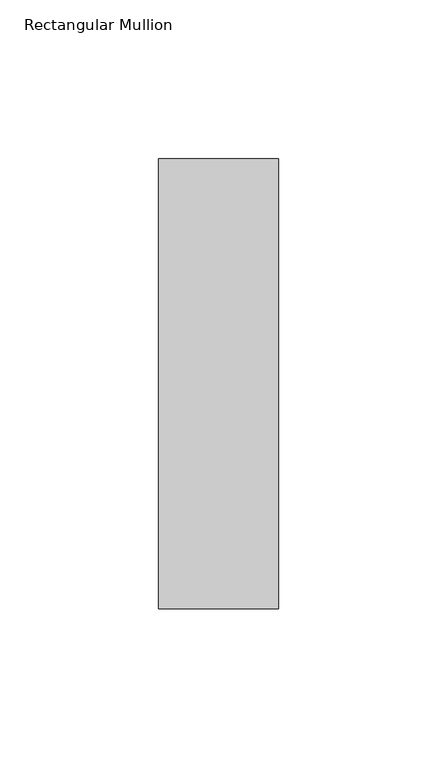
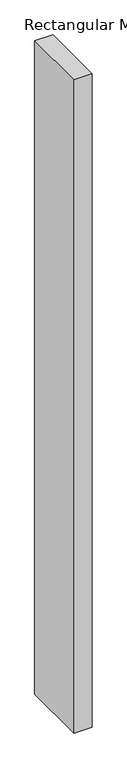
"""IFC4 building model written with IfcOpenShell, lengths in millimetres: member geometry, Rectangular Mullion : NLRS_21_CWM_hsb-regel 38x142_gen_rsf."""

from ifc_helpers import new_model, si_unit, frame, origin, place, context, project, spatial, polyline, outline, extrude, source, transform, mapped, element, save


def rectangular_mullion_dc0a3d83(model_context):
    return source(origin(), model_context, "Body", "SweptSolid", [
        extrude(outline(polyline([(-38.0, -71.0), (-38.0, 71.0), (0.0, 71.0), (0.0, -71.0), (-38.0, -71.0)])), frame((0.0, 0.0, -1440.0), z_axis=(0.0, 0.0, 1.0), x_axis=(1.0, 0.0, 0.0)), (0.0, 0.0, 1.0), 1440.0),
    ])


if __name__ == "__main__":
    model = new_model("IFC4")
    model_context = context("Model", 3, world=origin())
    ifc_project = project(units=[si_unit("LENGTHUNIT", "METRE", prefix="MILLI")], contexts=[model_context])
    site = spatial("IfcSite", under=ifc_project)
    building = spatial("IfcBuilding", under=site)
    placement = place(None, origin())
    rectangular_mullion_shape = rectangular_mullion_dc0a3d83(model_context)
    element("IfcMember", 1, ObjectType="Rectangular Mullion : NLRS_21_CWM_hsb-regel 38x142_gen_rsf", at=placement, inside=building, context=model_context, shape_type="MappedRepresentation", body=[
        mapped(rectangular_mullion_shape, transform((0.0, 0.0, 0.0), x_axis=(1.0, 0.0, 0.0), y_axis=(0.0, 1.0, 0.0), z_axis=(0.0, 0.0, 1.0))),
    ])
    save(model, "model.ifc")

# Revit data of these elements
# Type "Rectangular Mullion : NLRS_21_CWM_hsb-regel 38x142_gen_rsf"
#   Export Type to IFC As = "IfcWall"
#   Type IfcGUID = "07M7mRoiH1CR8m_RSKIwpF"
#   Assembly Code = "21.10"
#   built-in parameter 1007322 = 0.465879 (stored number, unit not read)
#   built-in parameter 1007321 = 0.062336 (stored number, unit not read)
#   built-in parameter 1007320 = 0.062336 (stored number, unit not read)
# Element 1 (IfcMember, "Rectangular Mullion : NLRS_21_CWM_hsb-regel 38x142_gen_rsf")
#   Materials on its faces: "NLRS_i2_hout naaldhout vuren_gen_rsf"
# Materials
#   "NLRS_i2_hout naaldhout vuren_gen_rsf": class "I - Hout", colour RGB 234 199 147, transparency 0, Keynote = "i2", Manufacturer = "Revit Standards Foundation", URL = "www.revitstandards.org", Description = "hout vuren", Cost = 0
